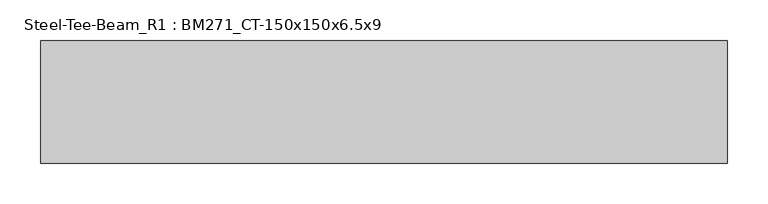
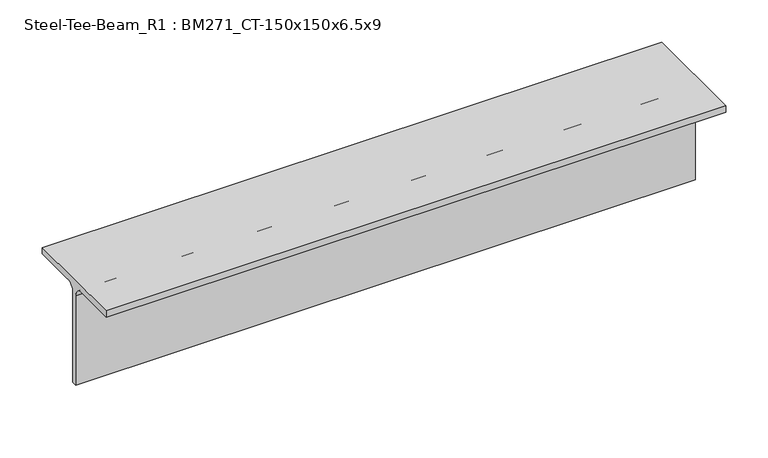
"""IFC4 building model written with IfcOpenShell, lengths in millimetres: member geometry, Steel-Tee-Beam_R1 : BM271_CT-150x150x6.5x9."""

from ifc_helpers import new_model, si_unit, point, frame, frame_2d, origin, place, context, project, spatial, polyline, circle_curve, trimmed, segment, composite_curve, outline, extrude, source, transform, mapped, element, save


def steel_tee_beam_r1_bm271_ct_150x150x6_5x9_52888b45(model_context):
    return source(origin(), model_context, "Body", "SweptSolid", [
        extrude(outline(composite_curve([segment(polyline([(-75.0, 75.0), (75.0, 75.0), (75.0, 66.0), (16.25, 66.0)]), True, "CONTINUOUS"), segment(trimmed(circle_curve(frame_2d((16.25, 53.0)), 13.0), [point((16.25, 66.0))], [point((3.25, 53.0))], True, "CARTESIAN"), True, "CONTINUOUS"), segment(polyline([(3.25, 53.0), (3.25, -75.0), (-3.25, -75.0), (-3.25, 53.0)]), True, "CONTINUOUS"), segment(trimmed(circle_curve(frame_2d((-16.25, 53.0)), 13.0), [point((-3.25, 53.0))], [point((-16.25, 66.0))], True, "CARTESIAN"), True, "CONTINUOUS"), segment(polyline([(-16.25, 66.0), (-75.0, 66.0), (-75.0, 75.0)]), True, "CONTINUOUS")], self_intersect=False)), frame((-341.5608007, 0.0, 0.0), z_axis=(1.0, 0.0, 0.0), x_axis=(0.0, 1.0, 0.0)), (0.0, 0.0, 1.0), 841.5608007),
    ])


if __name__ == "__main__":
    model = new_model("IFC4")
    model_context = context("Model", 3, world=origin())
    ifc_project = project(units=[si_unit("LENGTHUNIT", "METRE", prefix="MILLI")], contexts=[model_context])
    site = spatial("IfcSite", under=ifc_project)
    building = spatial("IfcBuilding", under=site)
    placement = place(None, origin())
    steel_tee_beam_r1_bm271_ct_150x150x6_5x9_shape = steel_tee_beam_r1_bm271_ct_150x150x6_5x9_52888b45(model_context)
    element("IfcMember", 1, ObjectType="Steel-Tee-Beam_R1 : BM271_CT-150x150x6.5x9", at=placement, inside=building, context=model_context, shape_type="MappedRepresentation", body=[
        mapped(steel_tee_beam_r1_bm271_ct_150x150x6_5x9_shape, transform((0.0, 0.0, 0.0), x_axis=(1.0, 0.0, 0.0), y_axis=(0.0, 1.0, 0.0), z_axis=(0.0, 0.0, 1.0))),
    ])
    save(model, "model.ifc")

# Revit data of these elements
# Type "Steel-Tee-Beam_R1 : BM271_CT-150x150x6.5x9"
#   Keynote = "CT-150x150x6.5x9"
#   Surface Area = 0.588841 m²/m
#   Section Area = 23.3904 cm²
#   Mass per Unit Length = 18.3614 kg/m
#   Length [instance default] = 1.5240 m
#   bf = 0.1500 m
#   d = 0.1500 m
#   k = 0.0220 m
#   r = 0.0130 m
#   tf = 0.0090 m
#   tw = 0.0065 m
#   hec_material4 [instance default] = none
#   hec_material3 [instance default] = none
#   hec_material2 [instance default] = none
#   hec_material1 [instance default] = none
#   Structural Material [instance default] = Steel, 45-345
#   Assembly Code = ""
# Element 1 (IfcMember, "Steel-Tee-Beam_R1 : BM271_CT-150x150x6.5x9")
#   Structural Material = none
# Materials
#   "Steel, 45-345": class "Metal", colour RGB 189 187 185, transparency 0, Description = "Steel 345 MPa", Cost = 0
